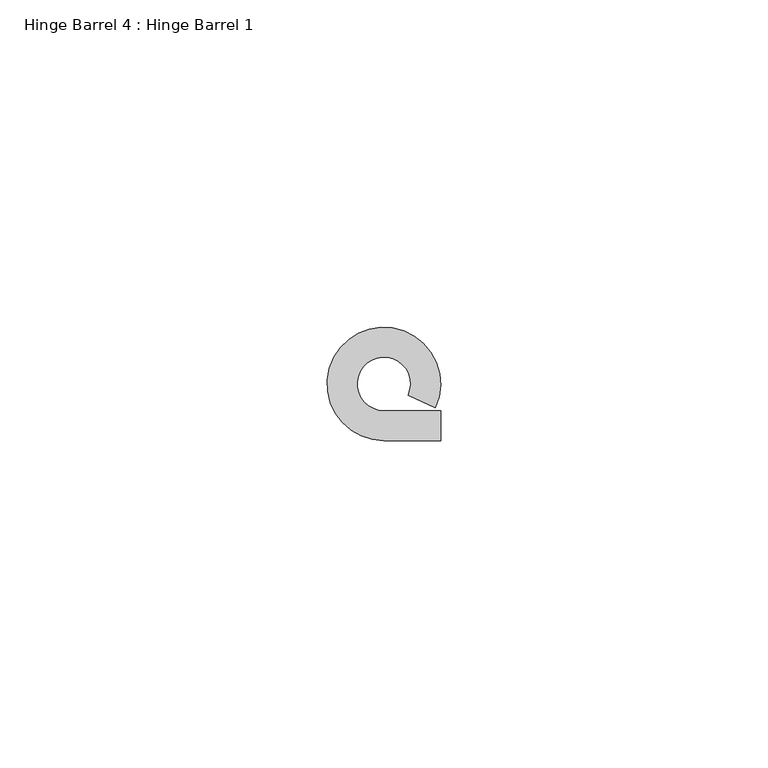
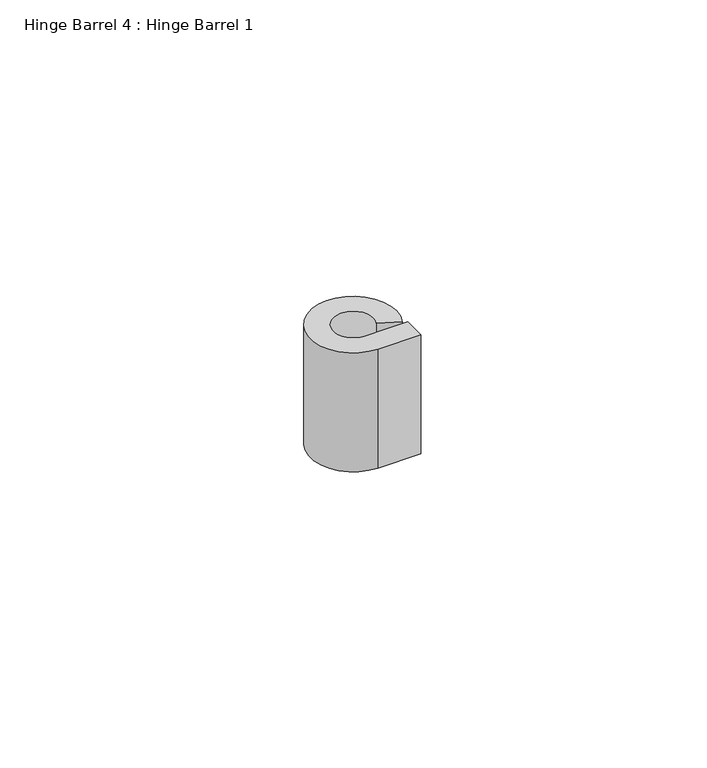
"""IFC4 building model written with IfcOpenShell, lengths in millimetres: proxy geometry, Hinge Barrel 4 : Hinge Barrel 1."""

from ifc_helpers import new_model, si_unit, point, frame, frame_2d, origin, place, context, project, spatial, polyline, circle_curve, trimmed, segment, composite_curve, outline, extrude, source, transform, mapped, element, save


def hinge_barrel_4_hinge_barrel_1_3de8cdcb(model_context):
    return source(origin(), model_context, "Body", "SweptSolid", [
        extrude(outline(composite_curve([segment(polyline([(587323.2214739, -531780.6943841), (587327.7934739, -531780.6943841), (587327.7934739, -531785.2584466), (587319.1320739, -531785.2584466)]), True, "CONTINUOUS"), segment(trimmed(circle_curve(frame_2d((587319.1320739, -531776.6049841)), 8.6534625), [point((587319.1320739, -531785.2584466))], [point((587326.986084, -531780.2377433))], False, "CARTESIAN"), True, "CONTINUOUS"), segment(polyline([(587326.986084, -531780.2377433), (587322.8436736, -531778.321731)]), True, "CONTINUOUS"), segment(trimmed(circle_curve(frame_2d((587319.1320739, -531776.6049841)), 4.0894), [point((587322.8436736, -531778.321731))], [point((587319.1320739, -531780.6943841))], True, "CARTESIAN"), True, "CONTINUOUS"), segment(polyline([(587319.1320739, -531780.6943841), (587323.2214739, -531780.6943841)]), True, "CONTINUOUS")], self_intersect=False)), frame((0.0, 0.0, 412.75), z_axis=(0.0, 0.0, 1.0), x_axis=(1.0, 0.0, 0.0)), (0.0, 0.0, 1.0), 25.4),
    ])


if __name__ == "__main__":
    model = new_model("IFC4")
    model_context = context("Model", 3, world=origin())
    ifc_project = project(units=[si_unit("LENGTHUNIT", "METRE", prefix="MILLI")], contexts=[model_context])
    site = spatial("IfcSite", under=ifc_project)
    building = spatial("IfcBuilding", under=site)
    placement = place(None, origin())
    hinge_barrel_4_hinge_barrel_1_shape = hinge_barrel_4_hinge_barrel_1_3de8cdcb(model_context)
    element("IfcBuildingElementProxy", 1, Name="Hinge Barrel 4 : Hinge Barrel 1", ObjectType="Hinge Barrel 4 : Hinge Barrel 1", at=placement, inside=building, context=model_context, shape_type="MappedRepresentation", body=[
        mapped(hinge_barrel_4_hinge_barrel_1_shape, transform((0.0, 0.0, 0.0), x_axis=(1.0, 0.0, 0.0), y_axis=(0.0, 1.0, 0.0), z_axis=(0.0, 0.0, 1.0))),
    ])
    save(model, "model.ifc")

# Revit data of these elements
# Element 1 (IfcBuildingElementProxy, "Hinge Barrel 4 : Hinge Barrel 1")
#   Materials on its faces: "6\"X6\" WELD-ON STL BUTT HINGE"
# Materials
#   "6\"X6\" WELD-ON STL BUTT HINGE": class "Metal", colour RGB 189 187 185, transparency 0, Description = "Carbon steel", Cost = 0
